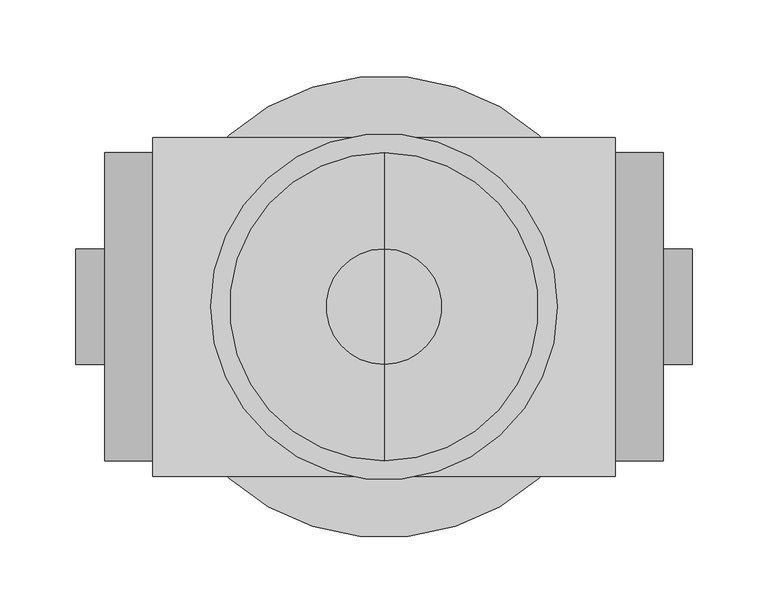
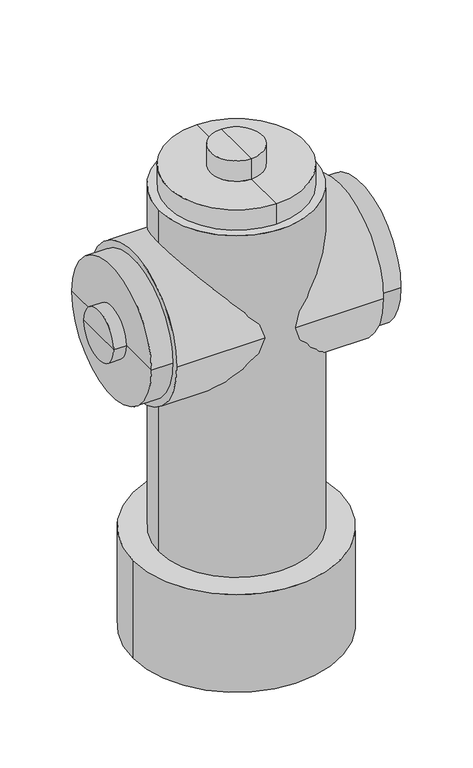
"""IFC4 building model written with IfcOpenShell, lengths in millimetres: proxy geometry, NLRS_90_GM_WPB_brandkraan_gen_rsf : brandkraan."""

from ifc_helpers import new_model, si_unit, point, frame, frame_2d, origin, origin_with_axes, origin_2d, place, context, project, spatial, circle_curve, trimmed, segment, composite_curve, outline, extrude, source, transform, mapped, element, save
from ifc_brep_helpers import plane_surface, cylinder_surface, advanced_brep


def generic_models_4a70fc30(model_context):
    return source(origin(), model_context, "Body", "SolidModel", [
        advanced_brep(
        [(0.0, 0.0, 558.8), (0.0, -101.6, 558.8), (0.0, 101.6, 558.8), (0.0, 38.1, 622.3), (0.0, -38.1, 622.3), (0.0, 0.0, 622.3), (0.0, 38.1, 590.55), (0.0, -38.1, 590.55), (0.0, 101.6, 590.55), (0.0, -101.6, 590.55)],
        [
            (0, 1),
            (1, 2, circle_curve(frame((0.0, 0.0, 558.8), z_axis=(0.0, 0.0, -1.0), x_axis=(0.0, -1.0, 0.0)), 101.6)),
            (2, 0),
            (2, 1, circle_curve(frame((0.0, 0.0, 558.8), z_axis=(0.0, 0.0, -1.0), x_axis=(0.0, -1.0, 0.0)), 101.6)),
            (3, 4, circle_curve(frame((0.0, 0.0, 622.3), z_axis=(0.0, 0.0, 1.0), x_axis=(0.0, -1.0, 0.0)), 38.1)),
            (4, 5),
            (5, 3),
            (4, 3, circle_curve(frame((0.0, 0.0, 622.3), z_axis=(0.0, 0.0, 1.0), x_axis=(0.0, -1.0, 0.0)), 38.1)),
            (6, 7, circle_curve(frame((0.0, 0.0, 590.55), z_axis=(0.0, 0.0, 1.0), x_axis=(0.0, -1.0, 0.0)), 38.1)),
            (7, 4),
            (3, 6),
            (7, 6, circle_curve(frame((0.0, 0.0, 590.55), z_axis=(0.0, 0.0, 1.0), x_axis=(0.0, -1.0, 0.0)), 38.1)),
            (8, 9, circle_curve(frame((0.0, 0.0, 590.55), z_axis=(0.0, 0.0, 1.0), x_axis=(0.0, -1.0, 0.0)), 101.6)),
            (9, 7),
            (6, 8),
            (9, 8, circle_curve(frame((0.0, 0.0, 590.55), z_axis=(0.0, 0.0, 1.0), x_axis=(0.0, -1.0, 0.0)), 101.6)),
            (1, 9),
            (8, 2),
        ],
        [
            plane_surface(frame((0.0, 0.0, 558.8), z_axis=(0.0, 0.0, -1.0), x_axis=(0.0, -1.0, 0.0))),
            plane_surface(frame((0.0, 0.0, 622.3), z_axis=(0.0, 0.0, 1.0), x_axis=(0.0, -1.0, 0.0))),
            cylinder_surface(frame((0.0, 0.0, 723.9), z_axis=(0.0, 0.0, -1.0), x_axis=(0.0, -1.0, 0.0)), 38.1),
            plane_surface(frame((0.0, 0.0, 590.55), z_axis=(0.0, 0.0, 1.0), x_axis=(0.0, -1.0, 0.0))),
            cylinder_surface(frame((0.0, 0.0, 723.9), z_axis=(0.0, 0.0, -1.0), x_axis=(0.0, -1.0, 0.0)), 101.6),
        ],
        [
            (0, [[1, 2, 3]]),
            (0, [[-3, 4, -1]]),
            (1, [[5, 6, 7]]),
            (1, [[8, -7, -6]]),
            (2, [[9, 10, -5, 11]]),
            (2, [[12, -11, -8, -10]]),
            (3, [[13, 14, -9, 15]]),
            (3, [[16, -15, -12, -14]]),
            (4, [[-2, 17, -13, 18]]),
            (4, [[-4, -18, -16, -17]]),
        ],
    ),
        advanced_brep(
        [(152.4, 0.0, 395.2562041), (152.4, 101.6, 395.2562041), (152.4, -101.6, 395.2562041), (203.2, -38.1, 395.2562041), (203.2, 38.1, 395.2562041), (203.2, 0.0, 395.2562041), (184.15, -38.1, 395.2562041), (184.15, 38.1, 395.2562041), (184.15, -101.6, 395.2562041), (184.15, 101.6, 395.2562041)],
        [
            (0, 1),
            (1, 2, circle_curve(frame((152.4, 0.0, 395.2562041), z_axis=(-1.0, 0.0, 0.0), x_axis=(0.0, 1.0, 0.0)), 101.6)),
            (2, 0),
            (2, 1, circle_curve(frame((152.4, 0.0, 395.2562041), z_axis=(-1.0, 0.0, 0.0), x_axis=(0.0, 1.0, 0.0)), 101.6)),
            (3, 4, circle_curve(frame((203.2, 0.0, 395.2562041), z_axis=(1.0, 0.0, 0.0), x_axis=(0.0, 1.0, 0.0)), 38.1)),
            (4, 5),
            (5, 3),
            (4, 3, circle_curve(frame((203.2, 0.0, 395.2562041), z_axis=(1.0, 0.0, 0.0), x_axis=(0.0, 1.0, 0.0)), 38.1)),
            (6, 7, circle_curve(frame((184.15, 0.0, 395.2562041), z_axis=(1.0, 0.0, 0.0), x_axis=(0.0, 1.0, 0.0)), 38.1)),
            (7, 4),
            (3, 6),
            (7, 6, circle_curve(frame((184.15, 0.0, 395.2562041), z_axis=(1.0, 0.0, 0.0), x_axis=(0.0, 1.0, 0.0)), 38.1)),
            (8, 9, circle_curve(frame((184.15, 0.0, 395.2562041), z_axis=(1.0, 0.0, 0.0), x_axis=(0.0, 1.0, 0.0)), 101.6)),
            (9, 7),
            (6, 8),
            (9, 8, circle_curve(frame((184.15, 0.0, 395.2562041), z_axis=(1.0, 0.0, 0.0), x_axis=(0.0, 1.0, 0.0)), 101.6)),
            (1, 9),
            (8, 2),
        ],
        [
            plane_surface(frame((152.4, 0.0, 395.2562041), z_axis=(-1.0, 0.0, 0.0), x_axis=(0.0, 1.0, 0.0))),
            plane_surface(frame((203.2, 0.0, 395.2562041), z_axis=(1.0, 0.0, 0.0), x_axis=(0.0, 1.0, 0.0))),
            cylinder_surface(frame((-254.0, 0.0, 395.2562041), z_axis=(-1.0, 0.0, 0.0), x_axis=(0.0, 1.0, 0.0)), 38.1),
            plane_surface(frame((184.15, 0.0, 395.2562041), z_axis=(1.0, 0.0, 0.0), x_axis=(0.0, 1.0, 0.0))),
            cylinder_surface(frame((-254.0, 0.0, 395.2562041), z_axis=(-1.0, 0.0, 0.0), x_axis=(0.0, 1.0, 0.0)), 101.6),
        ],
        [
            (0, [[1, 2, 3]]),
            (0, [[-3, 4, -1]]),
            (1, [[5, 6, 7]]),
            (1, [[8, -7, -6]]),
            (2, [[9, 10, -5, 11]]),
            (2, [[12, -11, -8, -10]]),
            (3, [[13, 14, -9, 15]]),
            (3, [[16, -15, -12, -14]]),
            (4, [[-2, 17, -13, 18]]),
            (4, [[-4, -18, -16, -17]]),
        ],
    ),
        advanced_brep(
        [(-184.15, -101.6, 395.2562041), (-184.15, 101.6, 395.2562041), (-152.4, 101.6, 395.2562041), (-152.4, -101.6, 395.2562041), (-184.15, -38.1, 395.2562041), (-184.15, 38.1, 395.2562041), (-203.2, -38.1, 395.2562041), (-203.2, 38.1, 395.2562041), (-203.2, 0.0, 395.2562041), (-152.4, 0.0, 395.2562041)],
        [
            (0, 1, circle_curve(frame((-184.15, 0.0, 395.2562041), z_axis=(1.0, 0.0, 0.0), x_axis=(0.0, 1.0, 0.0)), 101.6)),
            (1, 2),
            (2, 3, circle_curve(frame((-152.4, 0.0, 395.2562041), z_axis=(-1.0, 0.0, 0.0), x_axis=(0.0, 1.0, 0.0)), 101.6)),
            (3, 0),
            (1, 0, circle_curve(frame((-184.15, 0.0, 395.2562041), z_axis=(1.0, 0.0, 0.0), x_axis=(0.0, 1.0, 0.0)), 101.6)),
            (3, 2, circle_curve(frame((-152.4, 0.0, 395.2562041), z_axis=(-1.0, 0.0, 0.0), x_axis=(0.0, 1.0, 0.0)), 101.6)),
            (4, 5, circle_curve(frame((-184.15, 0.0, 395.2562041), z_axis=(1.0, 0.0, 0.0), x_axis=(0.0, 1.0, 0.0)), 38.1)),
            (5, 1),
            (0, 4),
            (5, 4, circle_curve(frame((-184.15, 0.0, 395.2562041), z_axis=(1.0, 0.0, 0.0), x_axis=(0.0, 1.0, 0.0)), 38.1)),
            (6, 7, circle_curve(frame((-203.2, 0.0, 395.2562041), z_axis=(1.0, 0.0, 0.0), x_axis=(0.0, 1.0, 0.0)), 38.1)),
            (7, 5),
            (4, 6),
            (7, 6, circle_curve(frame((-203.2, 0.0, 395.2562041), z_axis=(1.0, 0.0, 0.0), x_axis=(0.0, 1.0, 0.0)), 38.1)),
            (8, 7),
            (6, 8),
            (2, 9),
            (9, 3),
        ],
        [
            cylinder_surface(frame((-254.0, 0.0, 395.2562041), z_axis=(-1.0, 0.0, 0.0), x_axis=(0.0, 1.0, 0.0)), 101.6),
            plane_surface(frame((-184.15, 0.0, 395.2562041), z_axis=(-1.0, 0.0, 0.0), x_axis=(0.0, 1.0, 0.0))),
            cylinder_surface(frame((-254.0, 0.0, 395.2562041), z_axis=(-1.0, 0.0, 0.0), x_axis=(0.0, 1.0, 0.0)), 38.1),
            plane_surface(frame((-203.2, 0.0, 395.2562041), z_axis=(-1.0, 0.0, 0.0), x_axis=(0.0, 1.0, 0.0))),
            plane_surface(frame((-152.4, 0.0, 395.2562041), z_axis=(1.0, 0.0, 0.0), x_axis=(0.0, 1.0, 0.0))),
        ],
        [
            (0, [[1, 2, 3, 4]]),
            (0, [[5, -4, 6, -2]]),
            (1, [[7, 8, -1, 9]]),
            (1, [[10, -9, -5, -8]]),
            (2, [[11, 12, -7, 13]]),
            (2, [[14, -13, -10, -12]]),
            (3, [[15, -11, 16]]),
            (3, [[-16, -14, -15]]),
            (4, [[-3, 17, 18]]),
            (4, [[-6, -18, -17]]),
        ],
    ),
        extrude(outline(composite_curve([segment(trimmed(circle_curve(origin_2d(), 152.4), [point((-152.4, 0.0))], [point((152.4, 0.0))], False, "CARTESIAN"), True, "CONTINUOUS"), segment(trimmed(circle_curve(origin_2d(), 152.4), [point((152.4, 0.0))], [point((-152.4, 0.0))], False, "CARTESIAN"), True, "CONTINUOUS")], self_intersect=False)), frame((0.0, 0.0, -127.0), z_axis=(0.0, 0.0, 1.0), x_axis=(1.0, 0.0, 0.0)), (0.0, 0.0, 1.0), 152.4),
        extrude(outline(composite_curve([segment(trimmed(circle_curve(frame_2d((0.0, 395.2562041)), 111.76), [point((-111.76, 395.2562041))], [point((111.76, 395.2562041))], False, "CARTESIAN"), True, "CONTINUOUS"), segment(trimmed(circle_curve(frame_2d((0.0, 395.2562041)), 111.76), [point((111.76, 395.2562041))], [point((-111.76, 395.2562041))], False, "CARTESIAN"), True, "CONTINUOUS")], self_intersect=False)), frame((-152.4, 0.0, 0.0), z_axis=(1.0, 0.0, 0.0), x_axis=(0.0, 1.0, 0.0)), (0.0, 0.0, 1.0), 304.8),
        extrude(outline(composite_curve([segment(trimmed(circle_curve(origin_2d(), 114.3), [point((-114.3, 0.0))], [point((114.3, 0.0))], False, "CARTESIAN"), True, "CONTINUOUS"), segment(trimmed(circle_curve(origin_2d(), 114.3), [point((114.3, 0.0))], [point((-114.3, 0.0))], False, "CARTESIAN"), True, "CONTINUOUS")], self_intersect=False)), origin_with_axes(), (0.0, 0.0, 1.0), 558.8),
    ])


if __name__ == "__main__":
    model = new_model("IFC4")
    model_context = context("Model", 3, world=origin())
    ifc_project = project(units=[si_unit("LENGTHUNIT", "METRE", prefix="MILLI")], contexts=[model_context])
    site = spatial("IfcSite", under=ifc_project)
    building = spatial("IfcBuilding", under=site)
    placement = place(None, origin())
    generic_models_shape = generic_models_4a70fc30(model_context)
    element("IfcBuildingElementProxy", 1, Name="NLRS_90_GM_WPB_brandkraan_gen_rsf : brandkraan", ObjectType="NLRS_90_GM_WPB_brandkraan_gen_rsf : brandkraan", at=placement, inside=building, context=model_context, shape_type="MappedRepresentation", body=[
        mapped(generic_models_shape, transform((0.0, 0.0, 0.0), x_axis=(1.0, 0.0, 0.0), y_axis=(0.0, 1.0, 0.0), z_axis=(0.0, 0.0, 1.0))),
    ])
    save(model, "model.ifc")

# Revit data of these elements
# Type "NLRS_90_GM_WPB_brandkraan_gen_rsf : brandkraan"
#   Type IFC Predefined Type = "USERDEFINED"
#   Export Type to IFC As = "IfcGeographicElementType"
#   Type IfcGUID = "05J6pyYiTDtR2exmlhyPld"
#   IfcName[Type] = "brandkraan"
#   IfcDescription[Type] = "standaard brandkraan"
#   IfcObjectType[Type] = "HYDRANT"
#   IfcExportAs[Type] = "IfcGeographicElementType"
#   IfcExportType[Type] = "USERDEFINED"
#   NLRS_C_materiaal_afwerking [instance default] = ""
#   Model = "generiek"
#   Manufacturer = "Revit Standards Foundation"
#   Description = "standaard brandkraan"
#   Assembly Code = "90.71"
#   NLRS_S_gewicht [instance default] = 0.00 kg
#   NLRS_C_buiten [instance default] = yes
#   NLRS_C_materiaal = NLRS_h2_staal_gen_rsf
#   URL = ""
#   Default Elevation = 0
# Element 1 (IfcBuildingElementProxy, "NLRS_90_GM_WPB_brandkraan_gen_rsf : brandkraan")
#   Materials on its faces: "NLRS_h2_staal_gen_rsf"
# Materials
#   "NLRS_h2_staal_gen_rsf": class "H - Metaal", colour RGB 189 187 185, transparency 0, Keynote = "h2", Model = "generiek", Manufacturer = "Revit Standards Foundation", URL = "www.revitstandards.org", Description = "staal", Cost = 0
